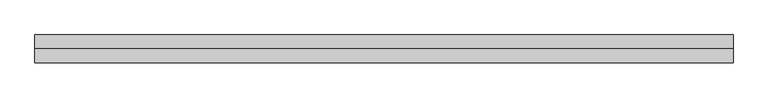
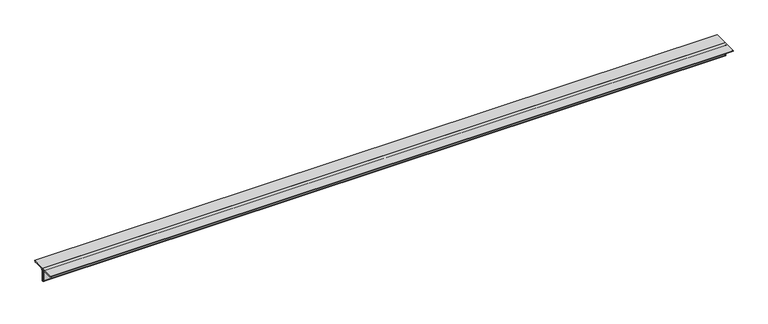
"""IFC4 building model written with IfcOpenShell, lengths in millimetres: member geometry, Steel Framing_2Ls_KS : H_SB_AR_S02_2Ls-100x100x10_VBR1."""

import ifcopenshell
import ifcopenshell.guid

model = None  # the IFC model being written
_history = None  # IfcOwnerHistory: only IFC2X3 demands one
_inside = {}  # id of a spatial element -> (the spatial element, [elements in it])
_under = {}  # id of a project, library or spatial element -> (it, [spatial elements below it])
_declared = {}  # id of a project -> (the project, [libraries it declares])
_typed = {}  # id of a type object -> (the type object, [elements of that type])
_made_of = {}  # id of a material, layer set ... -> (it, [elements and type objects made of it])


def new_model(schema):
    """Start an empty IFC model of exactly this schema.

    Asked for "IFC4X3", IfcOpenShell would pick the latest addendum, in which some entities
    have other attributes; the version numbers below select the first issue.
    IFC2X3 requires an IfcOwnerHistory on every rooted entity: one is made here for all.
    """
    global model, _history
    if schema == "IFC4X3":
        model = ifcopenshell.file(schema_version=(4, 3, 0, 0))
    else:
        model = ifcopenshell.file(schema=schema)
    _inside.clear()
    _under.clear()
    _declared.clear()
    _typed.clear()
    _made_of.clear()
    _history = None
    if model.schema == "IFC2X3":
        org = make("IfcOrganization", Name="unknown")
        user = make(
            "IfcPersonAndOrganization",
            ThePerson=make("IfcPerson", FamilyName="unknown"),
            TheOrganization=org,
        )
        app = make(
            "IfcApplication",
            ApplicationDeveloper=org,
            Version="unknown",
            ApplicationFullName="unknown",
            ApplicationIdentifier="unknown",
        )
        _history = make(
            "IfcOwnerHistory",
            OwningUser=user,
            OwningApplication=app,
            ChangeAction="ADDED",
            CreationDate=0,
        )
    return model


def make(cls, **values):
    """One entity of the class cls with the attributes given. An attribute that is None is left unset."""
    return model.create_entity(
        cls, **{name: value for name, value in values.items() if value is not None}
    )


def rooted(cls, **values):
    """An entity with a GlobalId (a new one), such as an element, a storey or a relation."""
    return make(cls, GlobalId=ifcopenshell.guid.new(), OwnerHistory=_history, **values)


def si_unit(unit_type, name, prefix=None):
    """IfcSIUnit, for example si_unit("LENGTHUNIT", "METRE", prefix="MILLI")."""
    return make("IfcSIUnit", UnitType=unit_type, Prefix=prefix, Name=name)


def assignment(units):
    """IfcUnitAssignment: the units of a project."""
    return None if units is None else make("IfcUnitAssignment", Units=units)


def point(xyz):
    """IfcCartesianPoint."""
    return None if xyz is None else make("IfcCartesianPoint", Coordinates=xyz)


def direction(xyz):
    """IfcDirection."""
    return None if xyz is None else make("IfcDirection", DirectionRatios=xyz)


def frame(location, z_axis=None, x_axis=None):
    """IfcAxis2Placement3D, a coordinate frame: its origin and axes. An axis left out is left unset."""
    return make(
        "IfcAxis2Placement3D",
        Location=point(location),
        Axis=direction(z_axis),
        RefDirection=direction(x_axis),
    )


def frame_2d(location, x_axis=None):
    """IfcAxis2Placement2D, a coordinate frame in the plane: its origin and x axis."""
    return make(
        "IfcAxis2Placement2D", Location=point(location), RefDirection=direction(x_axis)
    )


def origin():
    """The frame at (0, 0, 0) with its axes left unset."""
    return frame((0.0, 0.0, 0.0))


def place(relative_to, where):
    """IfcLocalPlacement: puts the frame where relative to a parent placement (None: the world)."""
    return make(
        "IfcLocalPlacement", PlacementRelTo=relative_to, RelativePlacement=where
    )


def context(
    kind, dimensions, precision=None, world=None, true_north=None, identifier=None
):
    """IfcGeometricRepresentationContext, for example the 3D "Model" context."""
    return make(
        "IfcGeometricRepresentationContext",
        ContextIdentifier=identifier,
        ContextType=kind,
        CoordinateSpaceDimension=dimensions,
        Precision=precision,
        WorldCoordinateSystem=world,
        TrueNorth=true_north,
    )


def project(units=None, contexts=None):
    """IfcProject with its units and contexts."""
    return rooted(
        "IfcProject",
        Name="project",
        RepresentationContexts=contexts,
        UnitsInContext=assignment(units),
    )


def spatial(cls, under=None, at=None, **own):
    """A site, building, storey or space (cls), placed at a placement, below another one or the project."""
    s = rooted(cls, ObjectPlacement=at, **own)
    if under is not None:
        _under.setdefault(under.id(), (under, []))[1].append(s)
    return s


def polyline(points):
    """IfcPolyline through the points."""
    return make("IfcPolyline", Points=[point(p) for p in points])


def circle_curve(where, radius):
    """IfcCircle in the frame where."""
    return make("IfcCircle", Position=where, Radius=radius)


def trimmed(basis, trim1, trim2, sense, master):
    """IfcTrimmedCurve: the piece of a basis curve between two trims."""
    return make(
        "IfcTrimmedCurve",
        BasisCurve=basis,
        Trim1=trim1,
        Trim2=trim2,
        SenseAgreement=sense,
        MasterRepresentation=master,
    )


def segment(curve, same_sense, transition):
    """IfcCompositeCurveSegment."""
    return make(
        "IfcCompositeCurveSegment",
        Transition=transition,
        SameSense=same_sense,
        ParentCurve=curve,
    )


def composite_curve(segments, self_intersect=None):
    """IfcCompositeCurve: segments joined end to end."""
    return make("IfcCompositeCurve", Segments=segments, SelfIntersect=self_intersect)


def outline(outer, holes=None, kind="AREA"):
    """IfcArbitraryClosedProfileDef: a profile drawn as a closed curve; with holes, ...WithVoids."""
    if holes is None:
        return make("IfcArbitraryClosedProfileDef", ProfileType=kind, OuterCurve=outer)
    return make(
        "IfcArbitraryProfileDefWithVoids",
        ProfileType=kind,
        OuterCurve=outer,
        InnerCurves=holes,
    )


def extrude(swept, where, along, depth):
    """IfcExtrudedAreaSolid: the profile swept, set in the frame where, extruded along a direction by depth."""
    return make(
        "IfcExtrudedAreaSolid",
        SweptArea=swept,
        Position=where,
        ExtrudedDirection=direction(along),
        Depth=depth,
    )


def shape(context_of_items, identifier, shape_type, items):
    """IfcShapeRepresentation: the items that make up one representation, for example the "Body"."""
    return make(
        "IfcShapeRepresentation",
        ContextOfItems=context_of_items,
        RepresentationIdentifier=identifier,
        RepresentationType=shape_type,
        Items=items,
    )


def source(mapping_origin, context_of_items, identifier, shape_type, items):
    """IfcRepresentationMap: a shape defined once, which mapped items show again and again."""
    return make(
        "IfcRepresentationMap",
        MappingOrigin=mapping_origin,
        MappedRepresentation=shape(context_of_items, identifier, shape_type, items),
    )


def transform(
    local_origin,
    x_axis=None,
    y_axis=None,
    z_axis=None,
    scale=None,
    scale2=None,
    scale3=None,
    uniform=True,
):
    """IfcCartesianTransformationOperator3D, or its non-uniform kind. x_axis, y_axis, z_axis: its Axis1, 2, 3."""
    if uniform:
        return make(
            "IfcCartesianTransformationOperator3D",
            Axis1=direction(x_axis),
            Axis2=direction(y_axis),
            LocalOrigin=point(local_origin),
            Scale=scale,
            Axis3=direction(z_axis),
        )
    return make(
        "IfcCartesianTransformationOperator3DnonUniform",
        Axis1=direction(x_axis),
        Axis2=direction(y_axis),
        LocalOrigin=point(local_origin),
        Scale=scale,
        Axis3=direction(z_axis),
        Scale2=scale2,
        Scale3=scale3,
    )


def mapped(mapping_source, mapping_target):
    """IfcMappedItem: shows the shape of a source again, moved by a transform."""
    return make(
        "IfcMappedItem", MappingSource=mapping_source, MappingTarget=mapping_target
    )


def made_of(thing, what):
    """Note that an element or type object is made of a material, layer set ...; save() writes the relation."""
    if what is not None:
        _made_of.setdefault(what.id(), (what, []))[1].append(thing)
    return thing


def element(
    cls,
    number,
    at=None,
    inside=None,
    cuts=None,
    type_object=None,
    material=None,
    context=None,
    identifier="Body",
    shape_type=None,
    held_by="IfcProductDefinitionShape",
    body=None,
    shapes=None,
    **own,
):
    """One element of the class cls, such as IfcWall. Its Tag is "e" and its number.

    at: its placement. inside: the storey or other place that contains it. cuts: it is an
    opening in that element (IfcRelVoidsElement). A single representation is given by context,
    identifier, shape_type and body (its items); several are given by shapes. held_by: the class
    of the entity that holds the representations. save() writes the other relations.
    """
    e = rooted(cls, Tag="e%d" % number, ObjectPlacement=at, **own)
    if body is not None:
        shapes = [shape(context, identifier, shape_type, body)]
    if shapes is not None:
        e.Representation = make(held_by, Representations=shapes)
    if inside is not None:
        _inside.setdefault(inside.id(), (inside, []))[1].append(e)
    if cuts is not None:
        rooted(
            "IfcRelVoidsElement", RelatingBuildingElement=cuts, RelatedOpeningElement=e
        )
    if type_object is not None:
        _typed.setdefault(type_object.id(), (type_object, []))[1].append(e)
    return made_of(e, material)


def aggregate(whole, parts):
    """IfcRelAggregates: a whole, such as a stair, and the parts it consists of."""
    return rooted("IfcRelAggregates", RelatingObject=whole, RelatedObjects=parts)


def save(model, path):
    """Write the relations noted so far, then the file.

    IfcRelAggregates (storeys below a building ...), IfcRelContainedInSpatialStructure (elements
    in a storey), IfcRelDefinesByType, IfcRelAssociatesMaterial and IfcRelDeclares: one each for
    every whole, place, type object, material and project.
    """
    for whole, parts in _under.values():
        aggregate(whole, parts)
    for where, things in _inside.values():
        rooted(
            "IfcRelContainedInSpatialStructure",
            RelatedElements=things,
            RelatingStructure=where,
        )
    for kind, things in _typed.values():
        rooted("IfcRelDefinesByType", RelatedObjects=things, RelatingType=kind)
    for what, things in _made_of.values():
        rooted("IfcRelAssociatesMaterial", RelatedObjects=things, RelatingMaterial=what)
    for by, libraries in _declared.values():
        rooted("IfcRelDeclares", RelatingContext=by, RelatedDefinitions=libraries)
    model.write(path)


def member_a8e375eb(model_context):
    return source(origin(), model_context, "Body", "SweptSolid", [
        extrude(outline(composite_curve([segment(polyline([(0.0, 28.2), (0.0, -71.8)]), True, "CONTINUOUS"), segment(trimmed(circle_curve(frame_2d((0.0, -61.8)), 10.0), [point((0.0, -71.8))], [point((-10.0, -61.8))], False, "CARTESIAN"), True, "CONTINUOUS"), segment(polyline([(-10.0, -61.8), (-10.0, 8.2)]), True, "CONTINUOUS"), segment(trimmed(circle_curve(frame_2d((-20.0, 8.2)), 10.0), [point((-10.0, 8.2))], [point((-20.0, 18.2))], True, "CARTESIAN"), True, "CONTINUOUS"), segment(polyline([(-20.0, 18.2), (-90.0, 18.2)]), True, "CONTINUOUS"), segment(trimmed(circle_curve(frame_2d((-90.0, 28.2)), 10.0), [point((-90.0, 18.2))], [point((-100.0, 28.2))], False, "CARTESIAN"), True, "CONTINUOUS"), segment(polyline([(-100.0, 28.2), (0.0, 28.2)]), True, "CONTINUOUS")], self_intersect=False)), frame((-2600.492603, 0.0, 0.0), z_axis=(1.0, 0.0, 0.0), x_axis=(0.0, 1.0, 0.0)), (0.0, 0.0, 1.0), 4992.4085104),
        extrude(outline(composite_curve([segment(polyline([(0.0, 28.2), (100.0, 28.2)]), True, "CONTINUOUS"), segment(trimmed(circle_curve(frame_2d((90.0, 28.2)), 10.0), [point((100.0, 28.2))], [point((90.0, 18.2))], False, "CARTESIAN"), True, "CONTINUOUS"), segment(polyline([(90.0, 18.2), (20.0, 18.2)]), True, "CONTINUOUS"), segment(trimmed(circle_curve(frame_2d((20.0, 8.2)), 10.0), [point((20.0, 18.2))], [point((10.0, 8.2))], True, "CARTESIAN"), True, "CONTINUOUS"), segment(polyline([(10.0, 8.2), (10.0, -61.8)]), True, "CONTINUOUS"), segment(trimmed(circle_curve(frame_2d((0.0, -61.8)), 10.0), [point((10.0, -61.8))], [point((0.0, -71.8))], False, "CARTESIAN"), True, "CONTINUOUS"), segment(polyline([(0.0, -71.8), (0.0, 28.2)]), True, "CONTINUOUS")], self_intersect=False)), frame((-2600.492603, 0.0, 0.0), z_axis=(1.0, 0.0, 0.0), x_axis=(0.0, 1.0, 0.0)), (0.0, 0.0, 1.0), 4992.4085104),
    ])


if __name__ == "__main__":
    model = new_model("IFC4")
    model_context = context("Model", 3, world=origin())
    ifc_project = project(units=[si_unit("LENGTHUNIT", "METRE", prefix="MILLI")], contexts=[model_context])
    site = spatial("IfcSite", under=ifc_project)
    building = spatial("IfcBuilding", under=site)
    placement = place(None, origin())
    member_shape = member_a8e375eb(model_context)
    element("IfcMember", 1, ObjectType="Steel Framing_2Ls_KS : H_SB_AR_S02_2Ls-100x100x10_VBR1", at=placement, inside=building, context=model_context, shape_type="MappedRepresentation", body=[
        mapped(member_shape, transform((0.0, 0.0, 0.0), x_axis=(1.0, 0.0, 0.0), y_axis=(0.0, 1.0, 0.0), z_axis=(0.0, 0.0, 1.0))),
    ])
    save(model, "model.ifc")

# Revit data of these elements
# Type "Steel Framing_2Ls_KS : H_SB_AR_S02_2Ls-100x100x10_VBR1"
#   Type Comments = "MAIN"
#   Type Mark = "VBR1"
#   H_SectionID = "2Ls-100x100x10"
#   Assembly Code = "B10"
#   Legs = "LLBB"
#   H_Ratio for Additional Steel Plate = 0.2
#   W = 0
#   Perimeter = 0.80 m²/m
#   Nominal Weight = 29.80 kgf/m
#   Length [instance default] = 1524 mm
#   Space = 0 mm
#   b = 100 mm
#   d = 100 mm
#   t = 10 mm
#   y = 28.2 mm
#   A = 0.0038 m²
#   Structural Material [instance default] = Steel, 45-345
# Element 1 (IfcMember, "Steel Framing_2Ls_KS : H_SB_AR_S02_2Ls-100x100x10_VBR1")
#   Materials on its faces: "Steel, 45-345"
# Materials
#   "Steel, 45-345": class "Metal", colour RGB 189 187 185, transparency 0, Description = "Steel 345 MPa", Cost = 0
